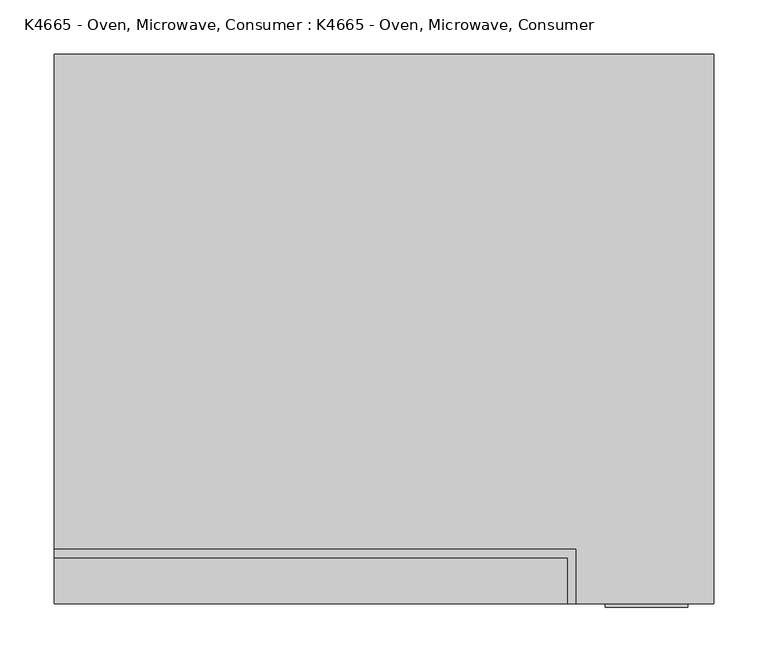
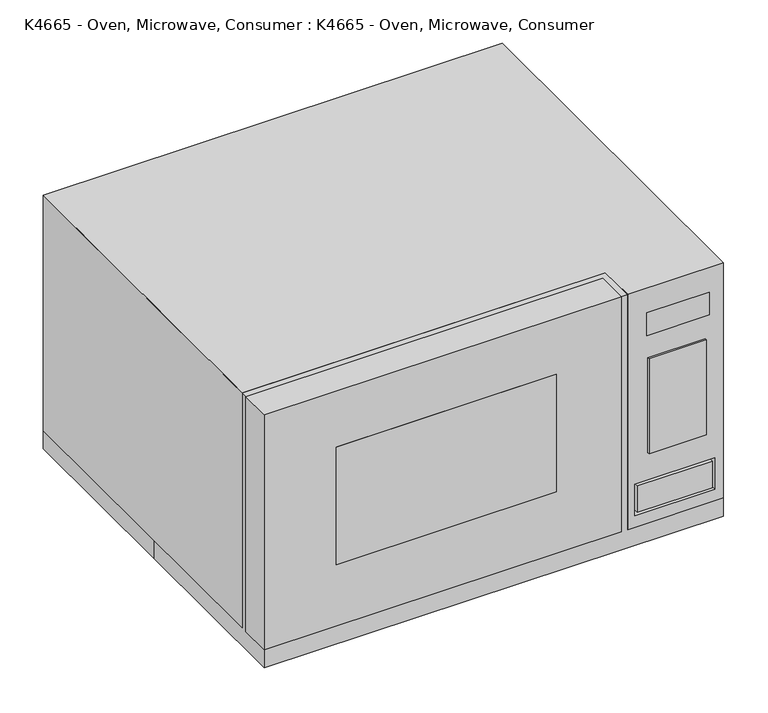
"""IFC4 building model written with IfcOpenShell, lengths in millimetres: proxy geometry, K4665 - Oven, Microwave, Consumer : K4665 - Oven, Microwave, Consumer."""

import ifcopenshell
import ifcopenshell.guid

model = None  # the IFC model being written
_history = None  # IfcOwnerHistory: only IFC2X3 demands one
_inside = {}  # id of a spatial element -> (the spatial element, [elements in it])
_under = {}  # id of a project, library or spatial element -> (it, [spatial elements below it])
_declared = {}  # id of a project -> (the project, [libraries it declares])
_typed = {}  # id of a type object -> (the type object, [elements of that type])
_made_of = {}  # id of a material, layer set ... -> (it, [elements and type objects made of it])


def new_model(schema):
    """Start an empty IFC model of exactly this schema.

    Asked for "IFC4X3", IfcOpenShell would pick the latest addendum, in which some entities
    have other attributes; the version numbers below select the first issue.
    IFC2X3 requires an IfcOwnerHistory on every rooted entity: one is made here for all.
    """
    global model, _history
    if schema == "IFC4X3":
        model = ifcopenshell.file(schema_version=(4, 3, 0, 0))
    else:
        model = ifcopenshell.file(schema=schema)
    _inside.clear()
    _under.clear()
    _declared.clear()
    _typed.clear()
    _made_of.clear()
    _history = None
    if model.schema == "IFC2X3":
        org = make("IfcOrganization", Name="unknown")
        user = make(
            "IfcPersonAndOrganization",
            ThePerson=make("IfcPerson", FamilyName="unknown"),
            TheOrganization=org,
        )
        app = make(
            "IfcApplication",
            ApplicationDeveloper=org,
            Version="unknown",
            ApplicationFullName="unknown",
            ApplicationIdentifier="unknown",
        )
        _history = make(
            "IfcOwnerHistory",
            OwningUser=user,
            OwningApplication=app,
            ChangeAction="ADDED",
            CreationDate=0,
        )
    return model


def make(cls, **values):
    """One entity of the class cls with the attributes given. An attribute that is None is left unset."""
    return model.create_entity(
        cls, **{name: value for name, value in values.items() if value is not None}
    )


def rooted(cls, **values):
    """An entity with a GlobalId (a new one), such as an element, a storey or a relation."""
    return make(cls, GlobalId=ifcopenshell.guid.new(), OwnerHistory=_history, **values)


def si_unit(unit_type, name, prefix=None):
    """IfcSIUnit, for example si_unit("LENGTHUNIT", "METRE", prefix="MILLI")."""
    return make("IfcSIUnit", UnitType=unit_type, Prefix=prefix, Name=name)


def assignment(units):
    """IfcUnitAssignment: the units of a project."""
    return None if units is None else make("IfcUnitAssignment", Units=units)


def point(xyz):
    """IfcCartesianPoint."""
    return None if xyz is None else make("IfcCartesianPoint", Coordinates=xyz)


def direction(xyz):
    """IfcDirection."""
    return None if xyz is None else make("IfcDirection", DirectionRatios=xyz)


def frame(location, z_axis=None, x_axis=None):
    """IfcAxis2Placement3D, a coordinate frame: its origin and axes. An axis left out is left unset."""
    return make(
        "IfcAxis2Placement3D",
        Location=point(location),
        Axis=direction(z_axis),
        RefDirection=direction(x_axis),
    )


def frame_2d(location, x_axis=None):
    """IfcAxis2Placement2D, a coordinate frame in the plane: its origin and x axis."""
    return make(
        "IfcAxis2Placement2D", Location=point(location), RefDirection=direction(x_axis)
    )


def origin():
    """The frame at (0, 0, 0) with its axes left unset."""
    return frame((0.0, 0.0, 0.0))


def origin_with_axes():
    """The frame at (0, 0, 0) with the z axis (0, 0, 1) and the x axis (1, 0, 0) written out."""
    return frame((0.0, 0.0, 0.0), z_axis=(0.0, 0.0, 1.0), x_axis=(1.0, 0.0, 0.0))


def place(relative_to, where):
    """IfcLocalPlacement: puts the frame where relative to a parent placement (None: the world)."""
    return make(
        "IfcLocalPlacement", PlacementRelTo=relative_to, RelativePlacement=where
    )


def context(
    kind, dimensions, precision=None, world=None, true_north=None, identifier=None
):
    """IfcGeometricRepresentationContext, for example the 3D "Model" context."""
    return make(
        "IfcGeometricRepresentationContext",
        ContextIdentifier=identifier,
        ContextType=kind,
        CoordinateSpaceDimension=dimensions,
        Precision=precision,
        WorldCoordinateSystem=world,
        TrueNorth=true_north,
    )


def project(units=None, contexts=None):
    """IfcProject with its units and contexts."""
    return rooted(
        "IfcProject",
        Name="project",
        RepresentationContexts=contexts,
        UnitsInContext=assignment(units),
    )


def spatial(cls, under=None, at=None, **own):
    """A site, building, storey or space (cls), placed at a placement, below another one or the project."""
    s = rooted(cls, ObjectPlacement=at, **own)
    if under is not None:
        _under.setdefault(under.id(), (under, []))[1].append(s)
    return s


def polyline(points):
    """IfcPolyline through the points."""
    return make("IfcPolyline", Points=[point(p) for p in points])


def circle_curve(where, radius):
    """IfcCircle in the frame where."""
    return make("IfcCircle", Position=where, Radius=radius)


def trimmed(basis, trim1, trim2, sense, master):
    """IfcTrimmedCurve: the piece of a basis curve between two trims."""
    return make(
        "IfcTrimmedCurve",
        BasisCurve=basis,
        Trim1=trim1,
        Trim2=trim2,
        SenseAgreement=sense,
        MasterRepresentation=master,
    )


def segment(curve, same_sense, transition):
    """IfcCompositeCurveSegment."""
    return make(
        "IfcCompositeCurveSegment",
        Transition=transition,
        SameSense=same_sense,
        ParentCurve=curve,
    )


def composite_curve(segments, self_intersect=None):
    """IfcCompositeCurve: segments joined end to end."""
    return make("IfcCompositeCurve", Segments=segments, SelfIntersect=self_intersect)


def outline(outer, holes=None, kind="AREA"):
    """IfcArbitraryClosedProfileDef: a profile drawn as a closed curve; with holes, ...WithVoids."""
    if holes is None:
        return make("IfcArbitraryClosedProfileDef", ProfileType=kind, OuterCurve=outer)
    return make(
        "IfcArbitraryProfileDefWithVoids",
        ProfileType=kind,
        OuterCurve=outer,
        InnerCurves=holes,
    )


def extrude(swept, where, along, depth):
    """IfcExtrudedAreaSolid: the profile swept, set in the frame where, extruded along a direction by depth."""
    return make(
        "IfcExtrudedAreaSolid",
        SweptArea=swept,
        Position=where,
        ExtrudedDirection=direction(along),
        Depth=depth,
    )


def faces_of(points, faces, orient=None, outer=None):
    """IfcFace entities. A face is a list of loops; a loop is a list of indices into points, from 0.

    orient and outer hold one flag for each loop. By default every Orientation is true, the
    first loop of a face is its IfcFaceOuterBound and the others are IfcFaceBound.
    """
    made = []
    for i, loops in enumerate(faces):
        bounds = []
        for j, loop in enumerate(loops):
            is_outer = j == 0 if outer is None else outer[i][j]
            bounds.append(
                make(
                    "IfcFaceOuterBound" if is_outer else "IfcFaceBound",
                    Bound=make("IfcPolyLoop", Polygon=[points[k] for k in loop]),
                    Orientation=True if orient is None else orient[i][j],
                )
            )
        made.append(make("IfcFace", Bounds=bounds))
    return made


def faceted_brep(points, faces, orient=None, outer=None, voids=None):
    """IfcFacetedBrep: a solid bounded by flat faces; with voids (closed shells), ...WithVoids."""
    shared = [point(p) for p in points]
    hull = make("IfcClosedShell", CfsFaces=faces_of(shared, faces, orient, outer))
    if voids is None:
        return make("IfcFacetedBrep", Outer=hull)
    return make(
        "IfcFacetedBrepWithVoids",
        Outer=hull,
        Voids=[
            make(cls, CfsFaces=faces_of(shared, fs, o, b)) for cls, fs, o, b in voids
        ],
    )


def shape(context_of_items, identifier, shape_type, items):
    """IfcShapeRepresentation: the items that make up one representation, for example the "Body"."""
    return make(
        "IfcShapeRepresentation",
        ContextOfItems=context_of_items,
        RepresentationIdentifier=identifier,
        RepresentationType=shape_type,
        Items=items,
    )


def source(mapping_origin, context_of_items, identifier, shape_type, items):
    """IfcRepresentationMap: a shape defined once, which mapped items show again and again."""
    return make(
        "IfcRepresentationMap",
        MappingOrigin=mapping_origin,
        MappedRepresentation=shape(context_of_items, identifier, shape_type, items),
    )


def transform(
    local_origin,
    x_axis=None,
    y_axis=None,
    z_axis=None,
    scale=None,
    scale2=None,
    scale3=None,
    uniform=True,
):
    """IfcCartesianTransformationOperator3D, or its non-uniform kind. x_axis, y_axis, z_axis: its Axis1, 2, 3."""
    if uniform:
        return make(
            "IfcCartesianTransformationOperator3D",
            Axis1=direction(x_axis),
            Axis2=direction(y_axis),
            LocalOrigin=point(local_origin),
            Scale=scale,
            Axis3=direction(z_axis),
        )
    return make(
        "IfcCartesianTransformationOperator3DnonUniform",
        Axis1=direction(x_axis),
        Axis2=direction(y_axis),
        LocalOrigin=point(local_origin),
        Scale=scale,
        Axis3=direction(z_axis),
        Scale2=scale2,
        Scale3=scale3,
    )


def mapped(mapping_source, mapping_target):
    """IfcMappedItem: shows the shape of a source again, moved by a transform."""
    return make(
        "IfcMappedItem", MappingSource=mapping_source, MappingTarget=mapping_target
    )


def made_of(thing, what):
    """Note that an element or type object is made of a material, layer set ...; save() writes the relation."""
    if what is not None:
        _made_of.setdefault(what.id(), (what, []))[1].append(thing)
    return thing


def element(
    cls,
    number,
    at=None,
    inside=None,
    cuts=None,
    type_object=None,
    material=None,
    context=None,
    identifier="Body",
    shape_type=None,
    held_by="IfcProductDefinitionShape",
    body=None,
    shapes=None,
    **own,
):
    """One element of the class cls, such as IfcWall. Its Tag is "e" and its number.

    at: its placement. inside: the storey or other place that contains it. cuts: it is an
    opening in that element (IfcRelVoidsElement). A single representation is given by context,
    identifier, shape_type and body (its items); several are given by shapes. held_by: the class
    of the entity that holds the representations. save() writes the other relations.
    """
    e = rooted(cls, Tag="e%d" % number, ObjectPlacement=at, **own)
    if body is not None:
        shapes = [shape(context, identifier, shape_type, body)]
    if shapes is not None:
        e.Representation = make(held_by, Representations=shapes)
    if inside is not None:
        _inside.setdefault(inside.id(), (inside, []))[1].append(e)
    if cuts is not None:
        rooted(
            "IfcRelVoidsElement", RelatingBuildingElement=cuts, RelatedOpeningElement=e
        )
    if type_object is not None:
        _typed.setdefault(type_object.id(), (type_object, []))[1].append(e)
    return made_of(e, material)


def aggregate(whole, parts):
    """IfcRelAggregates: a whole, such as a stair, and the parts it consists of."""
    return rooted("IfcRelAggregates", RelatingObject=whole, RelatedObjects=parts)


def save(model, path):
    """Write the relations noted so far, then the file.

    IfcRelAggregates (storeys below a building ...), IfcRelContainedInSpatialStructure (elements
    in a storey), IfcRelDefinesByType, IfcRelAssociatesMaterial and IfcRelDeclares: one each for
    every whole, place, type object, material and project.
    """
    for whole, parts in _under.values():
        aggregate(whole, parts)
    for where, things in _inside.values():
        rooted(
            "IfcRelContainedInSpatialStructure",
            RelatedElements=things,
            RelatingStructure=where,
        )
    for kind, things in _typed.values():
        rooted("IfcRelDefinesByType", RelatedObjects=things, RelatingType=kind)
    for what, things in _made_of.values():
        rooted("IfcRelAssociatesMaterial", RelatedObjects=things, RelatingMaterial=what)
    for by, libraries in _declared.values():
        rooted("IfcRelDeclares", RelatingContext=by, RelatedDefinitions=libraries)
    model.write(path)


def k4665_oven_microwave_consumer_k4665_oven_microwave_consumer_64c7f814(model_context):
    return source(origin(), model_context, "Body", "SolidModel", [
        extrude(outline(polyline([(280.7775556, -257.175), (204.5775556, -257.175), (204.5775556, -254.0), (280.7775556, -254.0), (280.7775556, -257.175)])), frame((0.0, 0.0, 124.244507), z_axis=(0.0, 0.0, 1.0), x_axis=(1.0, 0.0, 0.0)), (0.0, 0.0, 1.0), 133.35),
        extrude(outline(polyline([(286.1226613, -254.0), (203.5726613, -254.0), (203.5726613, -247.65), (286.1226613, -247.65), (286.1226613, -254.0)])), frame((0.0, 0.0, 288.87213), z_axis=(0.0, 0.0, 1.0), x_axis=(1.0, 0.0, 0.0)), (0.0, 0.0, 1.0), 31.75),
        extrude(outline(polyline([(82.9390055, -254.0), (-209.1609945, -254.0), (-209.1609945, -247.65), (82.9390055, -247.65), (82.9390055, -254.0)])), frame((0.0, 0.0, 111.4568552), z_axis=(0.0, 0.0, 1.0), x_axis=(1.0, 0.0, 0.0)), (0.0, 0.0, 1.0), 165.1),
        faceted_brep([(82.9390055, -235.0626171, 276.5568552), (-209.1609945, -235.0626171, 276.5568552), (-209.1609945, -235.0626171, 111.4568552), (82.9390055, -235.0626171, 111.4568552), (82.9390055, -254.0, 276.5568552), (-209.1609945, -254.0, 276.5568552), (-209.1609945, -254.0, 111.4568552), (82.9390055, -254.0, 111.4568552), (-304.8, -211.6756803, 355.6), (-304.8, -254.0, 355.6), (169.1942849, -254.0, 355.6), (169.1942849, -211.6756803, 355.6), (-304.8, -211.6756803, 25.4), (169.1942849, -211.6756803, 25.4), (169.1942849, -254.0, 25.4), (-304.8, -254.0, 25.4)], [[[0, 1, 2, 3]], [[1, 0, 4, 5]], [[2, 1, 5, 6]], [[3, 2, 6, 7]], [[0, 3, 7, 4]], [[8, 9, 10, 11]], [[12, 13, 14, 15]], [[9, 8, 12, 15]], [[10, 9, 15, 14], [5, 4, 7, 6]], [[11, 10, 14, 13]], [[8, 11, 13, 12]]]),
        extrude(outline(polyline([(-289.0486762, -203.2), (155.1090947, -203.2), (155.1090947, -211.6756803), (-289.0486762, -211.6756803), (-289.0486762, -203.2)])), frame((0.0, 0.0, 38.5670061), z_axis=(0.0, 0.0, 1.0), x_axis=(1.0, 0.0, 0.0)), (0.0, 0.0, 1.0), 304.3329939),
        faceted_brep([(286.1226613, -235.0626171, 320.62213), (203.5726613, -235.0626171, 320.62213), (203.5726613, -235.0626171, 288.87213), (286.1226613, -235.0626171, 288.87213), (286.1226613, -254.0, 320.62213), (203.5726613, -254.0, 320.62213), (203.5726613, -254.0, 288.87213), (286.1226613, -254.0, 288.87213), (293.5598712, -235.0626171, 41.6136485), (293.5598712, -235.0626171, 85.6060767), (187.4796019, -235.0626171, 85.6060767), (187.4796019, -235.0626171, 41.6136485), (190.7752155, -235.0626171, 82.3104632), (290.2642577, -235.0626171, 82.3104632), (290.2642577, -235.0626171, 44.909262), (190.7752155, -235.0626171, 44.909262), (187.4796019, -254.0, 85.6060767), (293.5598712, -254.0, 85.6060767), (190.7752155, -254.0, 82.3104632), (290.2642577, -254.0, 82.3104632), (290.2642577, -254.0, 44.909262), (190.7752155, -254.0, 44.909262), (187.4796019, -254.0, 41.6136485), (293.5598712, -254.0, 41.6136485), (304.8, 254.0, 355.6), (-304.8, 254.0, 355.6), (-304.8, -203.2, 355.6), (177.8, -203.2, 355.6), (177.8, -254.0, 355.6), (304.8, -254.0, 355.6), (304.8, 254.0, 25.4), (304.8, -254.0, 25.4), (177.8, -254.0, 25.4), (177.8, -203.2, 25.4), (-304.8, -203.2, 25.4), (-304.8, 254.0, 25.4)], [[[0, 1, 2, 3]], [[1, 0, 4, 5]], [[2, 1, 5, 6]], [[3, 2, 6, 7]], [[0, 3, 7, 4]], [[8, 9, 10, 11], [12, 13, 14, 15]], [[16, 10, 9, 17]], [[13, 12, 18, 19]], [[15, 14, 20, 21]], [[8, 11, 22, 23]], [[11, 10, 16, 22]], [[12, 15, 21, 18]], [[14, 13, 19, 20]], [[9, 8, 23, 17]], [[24, 25, 26, 27, 28, 29]], [[30, 31, 32, 33, 34, 35]], [[25, 24, 30, 35]], [[26, 25, 35, 34]], [[27, 26, 34, 33]], [[28, 27, 33, 32]], [[29, 28, 32, 31], [5, 4, 7, 6], [23, 22, 16, 17]], [[19, 18, 21, 20]], [[24, 29, 31, 30]]]),
        faceted_brep([(-304.8, 254.0, 355.6), (-304.8, 0.0, 355.6), (-304.8, -254.0, 355.6), (304.8, -254.0, 355.6), (304.8, 254.0, 355.6), (-304.8, 254.0, 0.0), (304.8, 254.0, 0.0), (304.8, -254.0, 0.0), (-304.8, -254.0, 0.0), (-304.8, 0.0, 0.0), (-209.1609945, -254.0, 276.5568552), (82.9390055, -254.0, 276.5568552), (82.9390055, -254.0, 111.4568552), (-209.1609945, -254.0, 111.4568552), (203.5726613, -254.0, 320.62213), (286.1226613, -254.0, 320.62213), (286.1226613, -254.0, 288.87213), (203.5726613, -254.0, 288.87213), (293.5598712, -254.0, 41.6136485), (187.4796019, -254.0, 41.6136485), (187.4796019, -254.0, 85.6060767), (293.5598712, -254.0, 85.6060767), (290.2642577, -254.0, 82.3104632), (190.7752155, -254.0, 82.3104632), (190.7752155, -254.0, 44.909262), (290.2642577, -254.0, 44.909262), (82.9390055, -235.0626171, 276.5568552), (-209.1609945, -235.0626171, 276.5568552), (-209.1609945, -235.0626171, 111.4568552), (82.9390055, -235.0626171, 111.4568552), (286.1226613, -235.0626171, 320.62213), (203.5726613, -235.0626171, 320.62213), (203.5726613, -235.0626171, 288.87213), (286.1226613, -235.0626171, 288.87213), (293.5598712, -235.0626171, 41.6136485), (293.5598712, -235.0626171, 85.6060767), (187.4796019, -235.0626171, 85.6060767), (187.4796019, -235.0626171, 41.6136485), (190.7752155, -235.0626171, 82.3104632), (290.2642577, -235.0626171, 82.3104632), (290.2642577, -235.0626171, 44.909262), (190.7752155, -235.0626171, 44.909262)], [[[0, 1, 2, 3, 4]], [[5, 6, 7, 8, 9]], [[1, 0, 5, 9]], [[2, 1, 9, 8]], [[3, 2, 8, 7], [10, 11, 12, 13], [14, 15, 16, 17], [18, 19, 20, 21]], [[22, 23, 24, 25]], [[4, 3, 7, 6]], [[0, 4, 6, 5]], [[26, 27, 28, 29]], [[27, 26, 11, 10]], [[28, 27, 10, 13]], [[29, 28, 13, 12]], [[26, 29, 12, 11]], [[30, 31, 32, 33]], [[31, 30, 15, 14]], [[32, 31, 14, 17]], [[33, 32, 17, 16]], [[30, 33, 16, 15]], [[34, 35, 36, 37], [38, 39, 40, 41]], [[20, 36, 35, 21]], [[39, 38, 23, 22]], [[41, 40, 25, 24]], [[34, 37, 19, 18]], [[37, 36, 20, 19]], [[38, 41, 24, 23]], [[40, 39, 22, 25]], [[35, 34, 18, 21]]]),
        extrude(outline(composite_curve([segment(trimmed(circle_curve(frame_2d((232.6731382, -121.4916445)), 25.4), [point((258.0731382, -121.4916445))], [point((207.2731382, -121.4916445))], False, "CARTESIAN"), True, "CONTINUOUS"), segment(trimmed(circle_curve(frame_2d((232.6731382, -121.4916445)), 25.4), [point((207.2731382, -121.4916445))], [point((258.0731382, -121.4916445))], False, "CARTESIAN"), True, "CONTINUOUS")], self_intersect=False)), origin_with_axes(), (0.0, 0.0, 1.0), 25.4),
        extrude(outline(composite_curve([segment(trimmed(circle_curve(frame_2d((-232.6731382, -121.4916445)), 25.4), [point((-258.0731382, -121.4916445))], [point((-207.2731382, -121.4916445))], False, "CARTESIAN"), True, "CONTINUOUS"), segment(trimmed(circle_curve(frame_2d((-232.6731382, -121.4916445)), 25.4), [point((-207.2731382, -121.4916445))], [point((-258.0731382, -121.4916445))], False, "CARTESIAN"), True, "CONTINUOUS")], self_intersect=False)), origin_with_axes(), (0.0, 0.0, 1.0), 25.4),
        extrude(outline(composite_curve([segment(trimmed(circle_curve(frame_2d((232.6731382, 183.3083555)), 25.4), [point((258.0731382, 183.3083555))], [point((207.2731382, 183.3083555))], False, "CARTESIAN"), True, "CONTINUOUS"), segment(trimmed(circle_curve(frame_2d((232.6731382, 183.3083555)), 25.4), [point((207.2731382, 183.3083555))], [point((258.0731382, 183.3083555))], False, "CARTESIAN"), True, "CONTINUOUS")], self_intersect=False)), origin_with_axes(), (0.0, 0.0, 1.0), 25.4),
        extrude(outline(composite_curve([segment(trimmed(circle_curve(frame_2d((-232.6731382, 183.3083555)), 25.4), [point((-258.0731382, 183.3083555))], [point((-207.2731382, 183.3083555))], False, "CARTESIAN"), True, "CONTINUOUS"), segment(trimmed(circle_curve(frame_2d((-232.6731382, 183.3083555)), 25.4), [point((-207.2731382, 183.3083555))], [point((-258.0731382, 183.3083555))], False, "CARTESIAN"), True, "CONTINUOUS")], self_intersect=False)), origin_with_axes(), (0.0, 0.0, 1.0), 25.4),
    ])


if __name__ == "__main__":
    model = new_model("IFC4")
    model_context = context("Model", 3, world=origin())
    ifc_project = project(units=[si_unit("LENGTHUNIT", "METRE", prefix="MILLI")], contexts=[model_context])
    site = spatial("IfcSite", under=ifc_project)
    building = spatial("IfcBuilding", under=site)
    placement = place(None, origin())
    k4665_oven_microwave_consumer_k4665_oven_microwave_consumer_shape = k4665_oven_microwave_consumer_k4665_oven_microwave_consumer_64c7f814(model_context)
    element("IfcBuildingElementProxy", 1, Name="K4665 - Oven, Microwave, Consumer : K4665 - Oven, Microwave, Consumer", ObjectType="K4665 - Oven, Microwave, Consumer : K4665 - Oven, Microwave, Consumer", at=placement, inside=building, context=model_context, shape_type="MappedRepresentation", body=[
        mapped(k4665_oven_microwave_consumer_k4665_oven_microwave_consumer_shape, transform((0.0, 0.0, 0.0), x_axis=(1.0, 0.0, 0.0), y_axis=(0.0, 1.0, 0.0), z_axis=(0.0, 0.0, 1.0))),
    ])
    save(model, "model.ifc")

# Revit data of these elements
# Type "K4665 - Oven, Microwave, Consumer : K4665 - Oven, Microwave, Consumer"
#   Watts2 = "0"
#   Watts1 = "1800"
#   Unit_Issue = "EA"
#   UTIL_6_Misc = "-"
#   UTIL_5_NonMedGas = "-"
#   UTIL_4_MiscGas = "-"
#   UTIL_3_MedGas = "-"
#   UTIL_2_Elec = "A"
#   UTIL_1_WaterDrain = "-"
#   Nomenclature = "Oven, Microwave, Consumer"
#   NSN = "7310"
#   Location [instance default] = ""
#   JSN = "K4665"
#   Fund_Source_VA = "-"
#   Fund_Source_Navy = "-"
#   Fund_Source_Army = "-"
#   Fund_Source_AF = "-"
#   ELEC_Volts2 = "0"
#   ELEC_Volts1 = "120"
#   ELEC_Phase2 = "0"
#   ELEC_Phase1 = "1"
#   ELEC_HertzSwitch = "0"
#   ELEC_HertzDependent = "-1"
#   ELEC_Hertz = "60"
#   ELEC_Amps2 = "0"
#   ELEC_Amps1 = "15"
#   DetailDescription = "Counter mounted microwave oven for average duty use. The exterior cabinet can be metal or heavy duty impact resistant plastic. The oven delivers instant energy for rapid heating, defrosting or prime cooking. The oven has touch pad controls, digital timer, power level selector and preprogrammed selectors for commonly cooked items. This oven is commonly found in staff lounges."
#   CAT_VA = "C"
#   CAT_Navy = "C"
#   CAT_IHS = "-"
#   CAT_Army = "C"
#   CAT_AF = "C"
#   BTUperhour = "0"
#   Weight_IP = 44
#   DIM_Width_IP = 2' - 0"
#   DIM_Height_IP = 1' - 2"
#   DIM_Depth_IP = 1' - 8"
# Element 1 (IfcBuildingElementProxy, "K4665 - Oven, Microwave, Consumer : K4665 - Oven, Microwave, Consumer")
#   Location = "NCWD1"
#   Materials on its faces: "EquipSpace", "Glass"
# Materials
#   "EquipSpace": class "Unassigned", colour RGB 221 217 195, transparency 0.5
#   "Glass": class "Glass", colour RGB 0 128 192, transparency 0.75
